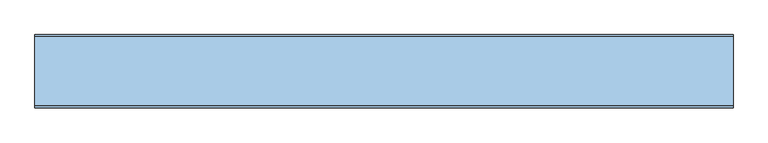
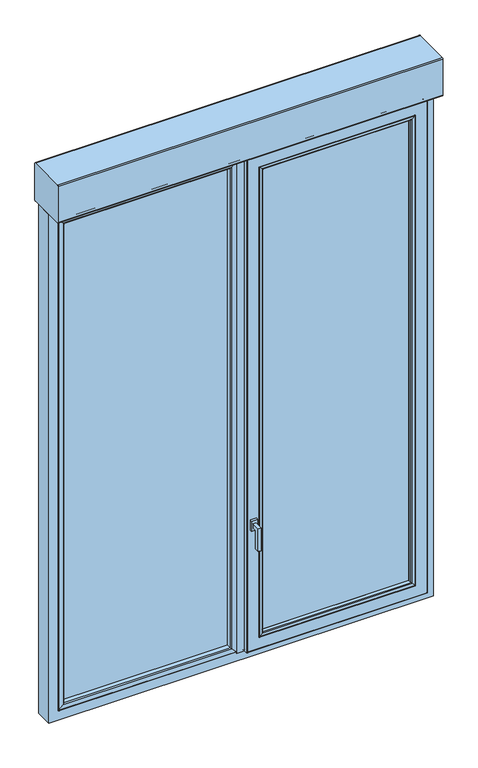
"""IFC4 building model written with IfcOpenShell, lengths in millimetres: window geometry, 2019_ES_Ventana_Replus_re80pvc301_11103_box_1-Hoja_Panel-Fijo-Lateral_con-Compacto : Salla."""

from ifc_helpers import new_model, si_unit, point, frame, frame_2d, origin, place, context, project, spatial, polyline, circle_curve, ellipse_curve, trimmed, segment, composite_curve, outline, extrude, source, transform, mapped, element, save
from ifc_brep_helpers import plane_surface, cylinder_surface, advanced_brep


def window_b88c883a(model_context):
    return source(origin(), model_context, "Body", "SolidModel", [
        extrude(outline(composite_curve([segment(polyline([(55.0, 3270.0), (-120.0, 3270.0)]), True, "CONTINUOUS"), segment(trimmed(circle_curve(frame_2d((-120.0, 3275.0)), 5.0), [point((-120.0, 3270.0))], [point((-125.0, 3275.0))], False, "CARTESIAN"), True, "CONTINUOUS"), segment(polyline([(-125.0, 3275.0), (-125.0, 3450.0)]), True, "CONTINUOUS"), segment(trimmed(circle_curve(frame_2d((-120.0, 3450.0)), 5.0), [point((-125.0, 3450.0))], [point((-120.0, 3455.0))], False, "CARTESIAN"), True, "CONTINUOUS"), segment(polyline([(-120.0, 3455.0), (55.0, 3455.0)]), True, "CONTINUOUS"), segment(trimmed(circle_curve(frame_2d((55.0, 3450.0)), 5.0), [point((55.0, 3455.0))], [point((60.0, 3450.0))], False, "CARTESIAN"), True, "CONTINUOUS"), segment(polyline([(60.0, 3450.0), (60.0, 3275.0)]), True, "CONTINUOUS"), segment(trimmed(circle_curve(frame_2d((55.0, 3275.0)), 5.0), [point((60.0, 3275.0))], [point((55.0, 3270.0))], False, "CARTESIAN"), True, "CONTINUOUS")], self_intersect=False)), frame((-880.0, 0.0, 0.0), z_axis=(1.0, 0.0, 0.0), x_axis=(0.0, 1.0, 0.0)), (0.0, 0.0, 1.0), 1760.0),
        extrude(outline(polyline([(-78.4999991, 1470.0), (-78.4999991, 1450.0), (-98.4999991, 1450.0), (-98.4999991, 1360.0), (-118.4999991, 1360.0), (-118.4999991, 1470.0), (-78.4999991, 1470.0)])), frame((38.5, 0.0, 0.0), z_axis=(1.0, 0.0, 0.0), x_axis=(0.0, 1.0, 0.0)), (0.0, 0.0, 1.0), 12.0),
        extrude(outline(polyline([(58.7312385, -78.4999991), (30.2687615, -78.4999991), (30.2687615, -68.4999991), (58.7312385, -68.4999991), (58.7312385, -78.4999991)])), frame((0.0, 0.0, 1435.217127), z_axis=(0.0, 0.0, 1.0), x_axis=(1.0, 0.0, 0.0)), (0.0, 0.0, 1.0), 49.565746),
        extrude(outline(polyline([(-37.0063666, 11.4999962), (-37.0063666, 7.4999962), (-814.1891471, 7.4999962), (-814.1891471, 11.4999962), (-37.0063666, 11.4999962)])), frame((0.0, 0.0, 875.6108529), z_axis=(0.0, 0.0, 1.0), x_axis=(1.0, 0.0, 0.0)), (0.0, 0.0, 1.0), 2328.7782941),
        extrude(outline(polyline([(-37.0063666, -6.5), (-37.0063666, -10.5), (-814.1891471, -10.5), (-814.1891471, -6.5), (-37.0063666, -6.5)])), frame((0.0, 0.0, 875.6108529), z_axis=(0.0, 0.0, 1.0), x_axis=(1.0, 0.0, 0.0)), (0.0, 0.0, 1.0), 2328.7782941),
        extrude(outline(polyline([(-37.0063666, -24.4999997), (-37.0063666, -28.4999997), (-814.1891471, -28.4999997), (-814.1891471, -24.4999997), (-37.0063666, -24.4999997)])), frame((0.0, 0.0, 875.6108529), z_axis=(0.0, 0.0, 1.0), x_axis=(1.0, 0.0, 0.0)), (0.0, 0.0, 1.0), 2328.7782941),
        advanced_brep(
        [(-22.1502489, -49.9816666, 3224.0497511), (-41.8192398, -49.2838062, 3204.3807602), (-41.8192398, -49.2838062, 875.6192398), (-22.1502489, -49.9816666, 855.9502489), (-46.4697163, -45.5846502, 3199.7302837), (-46.4697163, -45.5846502, 880.2697163), (-814.3807594, -49.2838062, 875.6192398), (-834.0497503, -49.9816666, 855.9502489), (-21.0, -48.871505, 3225.2), (-21.0, -48.871505, 854.8), (-51.0475336, -28.5000036, 3195.1524664), (-51.0475336, -28.5000036, 884.8475336), (-809.7302829, -45.5846502, 880.2697163), (-43.2922784, -28.5000036, 877.0922784), (-812.9077208, -28.5000036, 877.0922784), (-812.9077208, -28.5000036, 3202.9077216), (-43.2922784, -28.5000036, 3202.9077216), (-805.1524657, -28.5000036, 3195.1524664), (-805.1524657, -28.5000036, 884.8475336), (-35.4855, -36.306782, 3210.7145), (-35.4855, -36.306782, 869.2855), (-35.4855, -39.5069121, 3210.7145), (-35.4855, -39.5069121, 869.2855), (-820.7144993, -36.306782, 869.2855), (-21.0, -39.5069121, 854.8), (-835.1999993, -39.5069121, 854.8), (-835.1999993, -39.5069121, 3225.2), (-21.0, -39.5069121, 3225.2), (-820.7144993, -39.5069121, 3210.7145), (-820.7144993, -39.5069121, 869.2855), (-835.1999993, -48.871505, 854.8), (-814.3807594, -49.2838062, 3204.3807602), (-834.0497503, -49.9816666, 3224.0497511), (-809.7302829, -45.5846502, 3199.7302837), (-820.7144993, -36.306782, 3210.7145), (-835.1999993, -48.871505, 3225.2)],
        [
            (0, 1),
            (1, 2),
            (2, 3),
            (3, 0),
            (1, 4, ellipse_curve(frame((-41.6449168, -44.2918491, 3204.5550832), z_axis=(0.7071067811865475, 0.0, -0.7071067811865475), x_axis=(0.7071067811865474, 0.0, 0.7071067811865476)), 7.0639967, 4.995)),
            (4, 5),
            (5, 2, ellipse_curve(frame((-41.6449168, -44.2918491, 875.4449168), z_axis=(0.7071067811865475, 0.0, 0.7071067811865475), x_axis=(-0.7071067811865474, 0.0, 0.7071067811865476)), 7.0639967, 4.995)),
            (2, 6),
            (6, 7),
            (7, 3),
            (8, 0, ellipse_curve(frame((-22.1108601, -48.871505, 3224.0891399), z_axis=(0.7071067811865475, 0.0, -0.7071067811865475), x_axis=(0.7071067811865474, 0.0, 0.7071067811865476)), 1.5709935, 1.1108601)),
            (3, 9, ellipse_curve(frame((-22.1108601, -48.871505, 855.9108601), z_axis=(0.7071067811865475, 0.0, 0.7071067811865475), x_axis=(-0.7071067811865474, 0.0, 0.7071067811865476)), 1.5709935, 1.1108601)),
            (9, 8),
            (4, 10),
            (10, 11),
            (11, 5),
            (5, 12),
            (12, 6, ellipse_curve(frame((-814.5550824, -44.2918491, 875.4449168), z_axis=(0.7071067811865475, 0.0, -0.7071067811865475), x_axis=(0.7071067811865476, 0.0, 0.7071067811865474)), 7.0639967, 4.995)),
            (13, 14),
            (14, 15),
            (15, 16),
            (16, 13),
            (10, 17),
            (17, 18),
            (18, 11),
            (18, 12),
            (16, 19),
            (19, 20),
            (20, 13),
            (19, 21),
            (21, 22),
            (22, 20),
            (20, 23),
            (23, 14),
            (24, 25),
            (25, 26),
            (26, 27),
            (27, 24),
            (21, 28),
            (28, 29),
            (29, 22),
            (29, 23),
            (9, 24),
            (27, 8),
            (9, 30),
            (30, 25),
            (7, 30, ellipse_curve(frame((-834.0891391, -48.871505, 855.9108601), z_axis=(0.7071067811865475, 0.0, -0.7071067811865475), x_axis=(0.7071067811865476, 0.0, 0.7071067811865474)), 1.5709935, 1.1108601)),
            (6, 31),
            (31, 32),
            (32, 7),
            (12, 33),
            (33, 31, ellipse_curve(frame((-814.5550824, -44.2918491, 3204.5550832), z_axis=(-0.7071067811865475, 0.0, -0.7071067811865475), x_axis=(0.7071067811865474, 0.0, -0.7071067811865476)), 7.0639967, 4.995)),
            (17, 33),
            (23, 34),
            (34, 15),
            (28, 34),
            (30, 35),
            (35, 26),
            (32, 35, ellipse_curve(frame((-834.0891391, -48.871505, 3224.0891399), z_axis=(-0.7071067811865475, 0.0, -0.7071067811865475), x_axis=(0.7071067811865474, 0.0, -0.7071067811865476)), 1.5709935, 1.1108601)),
            (31, 1),
            (0, 32),
            (33, 4),
            (34, 19),
            (35, 8),
        ],
        [
            plane_surface(frame((-41.8192398, -49.2838062, 3204.3807602), z_axis=(-0.03545791932093311, -0.9993711702652975, 0.0), x_axis=(0.0, 0.0, -1.0))),
            cylinder_surface(frame((-41.6449168, -44.2918491, 3232.2), z_axis=(0.0, 0.0, 1.0), x_axis=(-1.0, 0.0, 0.0)), 4.995),
            plane_surface(frame((-41.8192398, -49.2838062, 875.6192398), z_axis=(0.0, -0.9993711702652976, 0.035457919320929884), x_axis=(-1.0, 0.0, 0.0))),
            cylinder_surface(frame((-22.1108601, -48.871505, 3232.2), z_axis=(0.0, 0.0, 1.0), x_axis=(-1.0, 0.0, 0.0)), 1.1108601),
            plane_surface(frame((-51.0475336, -28.5000036, 3195.1524664), z_axis=(-0.9659258262890619, -0.25881904510254483, 0.0), x_axis=(0.0, 0.0, -1.0))),
            cylinder_surface(frame((-14.0, -44.2918491, 875.4449168), z_axis=(1.0, 0.0, 0.0), x_axis=(0.0, 0.0, 1.0)), 4.995),
            plane_surface(frame((-812.9077208, -28.5000036, 3202.9077216), z_axis=(0.0, 1.0, 0.0), x_axis=(1.0, 0.0, 0.0))),
            plane_surface(frame((-51.0475336, -28.5000036, 884.8475336), z_axis=(0.0, -0.25881904510254794, 0.965925826289061), x_axis=(-1.0, 0.0, 0.0))),
            plane_surface(frame((-35.4855, -36.306782, 3210.7145), z_axis=(0.7071067811865617, 0.7071067811865334, 0.0), x_axis=(0.0, 0.0, -1.0))),
            plane_surface(frame((-35.4855, -39.5069121, 3210.7145), z_axis=(1.0, 0.0, 0.0), x_axis=(0.0, 0.0, -1.0))),
            plane_surface(frame((-35.4855, -36.306782, 869.2855), z_axis=(0.0, 0.7071067811865357, -0.7071067811865593), x_axis=(-1.0, 0.0, 0.0))),
            plane_surface(frame((-835.1999993, -39.5069121, 3225.2), z_axis=(0.0, 1.0, 0.0), x_axis=(1.0, 0.0, 0.0))),
            plane_surface(frame((-35.4855, -39.5069121, 869.2855), z_axis=(0.0, 0.0, -1.0), x_axis=(-1.0, 0.0, 0.0))),
            plane_surface(frame((-21.0, -46.2002121, 3225.2), z_axis=(1.0, 0.0, 0.0), x_axis=(0.0, 0.0, -1.0))),
            plane_surface(frame((-21.0, -46.2002121, 854.8), z_axis=(0.0, 0.0, -1.0), x_axis=(-1.0, 0.0, 0.0))),
            cylinder_surface(frame((-14.0, -48.871505, 855.9108601), z_axis=(1.0, 0.0, 0.0), x_axis=(0.0, 0.0, 1.0)), 1.1108601),
            plane_surface(frame((-814.3807594, -49.2838062, 875.6192398), z_axis=(0.03545791932092666, -0.9993711702652978, 0.0), x_axis=(0.0, 0.0, 1.0))),
            cylinder_surface(frame((-814.5550824, -44.2918491, 847.8), z_axis=(0.0, 0.0, -1.0), x_axis=(1.0, 0.0, 0.0)), 4.995),
            plane_surface(frame((-805.1524657, -28.5000036, 884.8475336), z_axis=(0.9659258262890602, -0.2588190451025511, 0.0), x_axis=(0.0, 0.0, 1.0))),
            plane_surface(frame((-820.7144993, -36.306782, 869.2855), z_axis=(-0.707106781186557, 0.707106781186538, 0.0), x_axis=(0.0, 0.0, 1.0))),
            plane_surface(frame((-820.7144993, -39.5069121, 869.2855), z_axis=(-1.0, 0.0, 0.0), x_axis=(0.0, 0.0, 1.0))),
            plane_surface(frame((-835.1999993, -46.2002121, 854.8), z_axis=(-1.0, 0.0, 0.0), x_axis=(0.0, 0.0, 1.0))),
            cylinder_surface(frame((-834.0891391, -48.871505, 847.8), z_axis=(0.0, 0.0, -1.0), x_axis=(1.0, 0.0, 0.0)), 1.1108601),
            plane_surface(frame((-814.3807594, -49.2838062, 3204.3807602), z_axis=(0.0, -0.9993711702652976, -0.035457919320929884), x_axis=(1.0, 0.0, 0.0))),
            cylinder_surface(frame((-842.1999993, -44.2918491, 3204.5550832), z_axis=(-1.0, 0.0, 0.0), x_axis=(0.0, 0.0, -1.0)), 4.995),
            plane_surface(frame((-805.1524657, -28.5000036, 3195.1524664), z_axis=(0.0, -0.258819045102548, -0.9659258262890611), x_axis=(1.0, 0.0, 0.0))),
            plane_surface(frame((-820.7144993, -36.306782, 3210.7145), z_axis=(0.0, 0.7071067811865357, 0.7071067811865593), x_axis=(1.0, 0.0, 0.0))),
            plane_surface(frame((-820.7144993, -39.5069121, 3210.7145), z_axis=(0.0, 0.0, 1.0), x_axis=(1.0, 0.0, 0.0))),
            plane_surface(frame((-835.1999993, -46.2002121, 3225.2), z_axis=(0.0, 0.0, 1.0), x_axis=(1.0, 0.0, 0.0))),
            cylinder_surface(frame((-842.1999993, -48.871505, 3224.0891399), z_axis=(-1.0, 0.0, 0.0), x_axis=(0.0, 0.0, -1.0)), 1.1108601),
        ],
        [
            (0, [[1, 2, 3, 4]]),
            (1, [[5, 6, 7, -2]]),
            (2, [[-3, 8, 9, 10]]),
            (3, [[11, -4, 12, 13]]),
            (4, [[14, 15, 16, -6]]),
            (5, [[-7, 17, 18, -8]]),
            (6, [[19, 20, 21, 22], [23, 24, 25, -15]]),
            (7, [[-16, -25, 26, -17]]),
            (8, [[27, 28, 29, -22]]),
            (9, [[30, 31, 32, -28]]),
            (10, [[-29, 33, 34, -19]]),
            (11, [[35, 36, 37, 38], [39, 40, 41, -31]]),
            (12, [[-32, -41, 42, -33]]),
            (13, [[-13, 43, -38, 44]]),
            (14, [[-43, 45, 46, -35]]),
            (15, [[-12, -10, 47, -45]]),
            (16, [[-9, 48, 49, 50]]),
            (17, [[-18, 51, 52, -48]]),
            (18, [[-26, -24, 53, -51]]),
            (19, [[-34, 54, 55, -20]]),
            (20, [[-42, -40, 56, -54]]),
            (21, [[-46, 57, 58, -36]]),
            (22, [[-47, -50, 59, -57]]),
            (23, [[-49, 60, -1, 61]]),
            (24, [[-52, 62, -5, -60]]),
            (25, [[-53, -23, -14, -62]]),
            (26, [[-55, 63, -27, -21]]),
            (27, [[-56, -39, -30, -63]]),
            (28, [[-58, 64, -44, -37]]),
            (29, [[-59, -61, -11, -64]]),
        ],
    ),
        extrude(outline(polyline([(3167.0, 777.1999993), (3167.0, 81.0), (912.8, 81.0), (912.8, 777.1999993), (3167.0, 777.1999993)]), holes=[polyline([(920.8, 769.1999993), (920.8, 89.0), (3159.0, 89.0), (3159.0, 769.1999993), (920.8, 769.1999993)])]), frame((0.0, -27.0000002, 0.0), z_axis=(0.0, 1.0, 0.0), x_axis=(0.0, 0.0, 1.0)), (0.0, 0.0, 1.0), 16.0000002),
        extrude(outline(polyline([(3167.0, 777.1999993), (3167.0, 81.0), (912.8, 81.0), (912.8, 777.1999993), (3167.0, 777.1999993)]), holes=[polyline([(920.8, 769.1999993), (920.8, 89.0), (3159.0, 89.0), (3159.0, 769.1999993), (920.8, 769.1999993)])]), frame((0.0, -47.0000002, 0.0), z_axis=(0.0, 1.0, 0.0), x_axis=(0.0, 0.0, 1.0)), (0.0, 0.0, 1.0), 16.0000002),
        extrude(outline(polyline([(3198.3891471, -43.0063666), (3198.3891471, -808.1891471), (881.8608529, -808.1891471), (881.8608529, -43.0063666), (3198.3891471, -43.0063666)]), holes=[polyline([(889.8608529, -51.0063666), (889.8608529, -800.1891471), (3190.3891471, -800.1891471), (3190.3891471, -51.0063666), (889.8608529, -51.0063666)])]), frame((0.0, -24.5, 0.0), z_axis=(0.0, 1.0, 0.0), x_axis=(0.0, 0.0, 1.0)), (0.0, 0.0, 1.0), 14.0),
        extrude(outline(polyline([(3198.3891471, -43.0063666), (3198.3891471, -808.1891471), (881.8608529, -808.1891471), (881.8608529, -43.0063666), (3198.3891471, -43.0063666)]), holes=[polyline([(889.8608529, -51.0063666), (889.8608529, -800.1891471), (3190.3891471, -800.1891471), (3190.3891471, -51.0063666), (889.8608529, -51.0063666)])]), frame((0.0, -6.5, 0.0), z_axis=(0.0, 1.0, 0.0), x_axis=(0.0, 0.0, 1.0)), (0.0, 0.0, 1.0), 14.0),
        advanced_brep(
        [(48.1911809, 11.5, 3200.2), (48.1911809, 11.5, 879.8), (48.1911809, -11.9999991, 879.8), (48.1911809, -11.9999991, 3200.2), (810.1999993, 11.5, 3200.2), (810.1999993, 11.5, 879.8), (88.2020856, 11.5, 919.8109047), (770.1890945, 11.5, 919.8109047), (770.1890945, 11.5, 3160.1890953), (88.2020856, 11.5, 3160.1890953), (810.1999993, -11.9999991, 879.8), (35.1911809, -11.9999991, 3213.2), (823.1999993, -11.9999991, 3213.2), (823.1999993, -11.9999991, 866.8), (35.1911809, -11.9999991, 866.8), (810.1999993, -11.9999991, 3200.2), (35.1911809, -50.0, 866.8), (35.1911809, -50.0, 3213.2), (823.1999993, -50.0, 866.8), (15.1911809, -50.0, 3233.2), (843.1999993, -50.0, 3233.2), (843.1999993, -50.0, 846.8), (15.1911809, -50.0, 846.8), (823.1999993, -50.0, 3213.2), (15.1911809, -65.4999991, 3233.2), (15.1911809, -65.4999991, 846.8), (843.1999993, -65.4999991, 846.8), (18.1911809, -68.4999991, 3230.2), (18.1911809, -68.4999991, 849.8), (840.1999993, -68.4999991, 849.8), (840.1999993, -68.4999991, 3230.2), (70.9541209, -68.4999991, 3177.43706), (787.4370593, -68.4999991, 3177.43706), (787.4370593, -68.4999991, 902.56294), (70.9541209, -68.4999991, 902.56294), (72.1911809, -67.2629391, 3176.2), (72.1911809, -67.2629391, 903.8), (786.1999993, -67.2629391, 903.8), (72.7423375, -67.7951848, 3175.6488434), (72.7423375, -67.7951848, 904.3511566), (785.6488427, -67.7951848, 904.3511566), (85.7676831, -67.3403297, 3162.6234978), (85.7676831, -67.3403297, 917.3765022), (772.6234971, -67.3403297, 917.3765022), (89.4917884, -64.3780426, 3158.8993925), (89.4917884, -64.3780426, 921.1006075), (768.8993918, -64.3780426, 921.1006075), (92.8970803, -51.6693201, 3155.4941006), (92.8970803, -51.6693201, 924.5058994), (765.4940999, -51.6693201, 924.5058994), (92.3834932, -51.0000003, 3156.0076877), (92.3834932, -51.0000003, 923.9923123), (766.007687, -51.0000003, 923.9923123), (81.1911809, -51.0000003, 3167.2), (777.1999993, -51.0000003, 3167.2), (777.1999993, -51.0000003, 912.8), (81.1911809, -51.0000003, 912.8), (766.007687, -51.0000003, 3156.0076877), (81.1911809, -56.4999995, 3167.2), (81.1911809, -56.4999995, 912.8), (777.1999993, -56.4999995, 912.8), (69.1911809, -56.4999995, 3179.2), (789.1999993, -56.4999995, 3179.2), (789.1999993, -56.4999995, 900.8), (69.1911809, -56.4999995, 900.8), (777.1999993, -56.4999995, 3167.2), (69.1911809, -25.6153717, 3179.2), (69.1911809, -25.6153717, 900.8), (789.1999993, -25.6153717, 900.8), (66.574961, -6.9999997, 3181.8162199), (66.574961, -6.9999997, 898.1837801), (791.8162192, -6.9999997, 898.1837801), (791.8162192, -6.9999997, 3181.8162199), (87.1911809, -6.9999997, 3161.2), (771.1999993, -6.9999997, 3161.2), (771.1999993, -6.9999997, 918.8), (87.1911809, -6.9999997, 918.8), (87.1911809, -3.0000033, 3161.2), (87.1911809, -3.0000033, 918.8), (771.1999993, -3.0000033, 918.8), (771.1999993, -3.0000033, 3161.2), (93.7172496, -3.0000033, 3154.6739313), (764.6739305, -3.0000033, 3154.6739313), (764.6739305, -3.0000033, 925.3260687), (93.7172496, -3.0000033, 925.3260687), (94.2153834, -2.3508228, 3154.1757976), (94.2153834, -2.3508228, 925.8242024), (764.1757968, -2.3508228, 925.8242024), (91.0998631, 9.2764571, 3157.2913178), (91.0998631, 9.2764571, 922.7086822), (767.2913171, 9.2764571, 922.7086822), (843.1999993, -65.4999991, 3233.2), (786.1999993, -67.2629391, 3176.2), (785.6488427, -67.7951848, 3175.6488434), (772.6234971, -67.3403297, 3162.6234978), (768.8993918, -64.3780426, 3158.8993925), (765.4940999, -51.6693201, 3155.4941006), (789.1999993, -25.6153717, 3179.2), (764.1757968, -2.3508228, 3154.1757976), (767.2913171, 9.2764571, 3157.2913178)],
        [
            (0, 1),
            (1, 2),
            (2, 3),
            (3, 0),
            (0, 4),
            (4, 5),
            (5, 1),
            (6, 7),
            (7, 8),
            (8, 9),
            (9, 6),
            (5, 10),
            (10, 2),
            (11, 12),
            (12, 13),
            (13, 14),
            (14, 11),
            (10, 15),
            (15, 3),
            (14, 16),
            (16, 17),
            (17, 11),
            (13, 18),
            (18, 16),
            (19, 20),
            (20, 21),
            (21, 22),
            (22, 19),
            (18, 23),
            (23, 17),
            (24, 19),
            (22, 25),
            (25, 24),
            (21, 26),
            (26, 25),
            (27, 24, ellipse_curve(frame((18.1911809, -65.4999991, 3230.2), z_axis=(-0.7071067811865475, 0.0, -0.7071067811865475), x_axis=(-0.7071067811865474, 0.0, 0.7071067811865476)), 4.2426407, 3.0)),
            (25, 28, ellipse_curve(frame((18.1911809, -65.4999991, 849.8), z_axis=(-0.7071067811865475, 0.0, 0.7071067811865475), x_axis=(0.7071067811865474, 0.0, 0.7071067811865476)), 4.2426407, 3.0)),
            (28, 27),
            (26, 29, ellipse_curve(frame((840.1999993, -65.4999991, 849.8), z_axis=(-0.7071067811865475, 0.0, -0.7071067811865475), x_axis=(-0.7071067811865476, 0.0, 0.7071067811865474)), 4.2426407, 3.0)),
            (29, 28),
            (29, 30),
            (30, 27),
            (31, 32),
            (32, 33),
            (33, 34),
            (34, 31),
            (35, 31, ellipse_curve(frame((70.9541209, -67.2629391, 3177.43706), z_axis=(-0.7071067811865475, 0.0, -0.7071067811865475), x_axis=(-0.7071067811865474, 0.0, 0.7071067811865476)), 1.7494671, 1.23706)),
            (34, 36, ellipse_curve(frame((70.9541209, -67.2629391, 902.56294), z_axis=(-0.7071067811865475, 0.0, 0.7071067811865475), x_axis=(0.7071067811865474, 0.0, 0.7071067811865476)), 1.7494671, 1.23706)),
            (36, 35),
            (33, 37, ellipse_curve(frame((787.4370593, -67.2629391, 902.56294), z_axis=(-0.7071067811865475, 0.0, -0.7071067811865475), x_axis=(-0.7071067811865476, 0.0, 0.7071067811865474)), 1.7494671, 1.23706)),
            (37, 36),
            (38, 35, ellipse_curve(frame((72.7237511, -67.2629391, 3175.6674299), z_axis=(-0.7071067811865475, 0.0, -0.7071067811865475), x_axis=(-0.7071067811865474, 0.0, 0.7071067811865476)), 0.7531679, 0.5325701)),
            (36, 39, ellipse_curve(frame((72.7237511, -67.2629391, 904.3325701), z_axis=(-0.7071067811865475, 0.0, 0.7071067811865475), x_axis=(0.7071067811865474, 0.0, 0.7071067811865476)), 0.7531679, 0.5325701)),
            (39, 38),
            (37, 40, ellipse_curve(frame((785.6674291, -67.2629391, 904.3325701), z_axis=(-0.7071067811865475, 0.0, -0.7071067811865475), x_axis=(-0.7071067811865476, 0.0, 0.7071067811865474)), 0.7531679, 0.5325701)),
            (40, 39),
            (41, 38),
            (39, 42),
            (42, 41),
            (40, 43),
            (43, 42),
            (44, 41, ellipse_curve(frame((85.6280851, -63.3427664, 3162.7630958), z_axis=(-0.7071067811865475, 0.0, -0.7071067811865475), x_axis=(-0.7071067811865474, 0.0, 0.7071067811865476)), 5.6568542, 4.0)),
            (42, 45, ellipse_curve(frame((85.6280851, -63.3427664, 917.2369042), z_axis=(-0.7071067811865475, 0.0, 0.7071067811865475), x_axis=(0.7071067811865474, 0.0, 0.7071067811865476)), 5.6568542, 4.0)),
            (45, 44),
            (43, 46, ellipse_curve(frame((772.7630951, -63.3427664, 917.2369042), z_axis=(-0.7071067811865475, 0.0, -0.7071067811865475), x_axis=(-0.7071067811865476, 0.0, 0.7071067811865474)), 5.6568542, 4.0)),
            (46, 45),
            (47, 44),
            (45, 48),
            (48, 47),
            (46, 49),
            (49, 48),
            (50, 47, ellipse_curve(frame((92.3834932, -51.5317048, 3156.0076877), z_axis=(-0.7071067811865475, 0.0, -0.7071067811865475), x_axis=(-0.7071067811865474, 0.0, 0.7071067811865476)), 0.7519437, 0.5317045)),
            (48, 51, ellipse_curve(frame((92.3834932, -51.5317048, 923.9923123), z_axis=(-0.7071067811865475, 0.0, 0.7071067811865475), x_axis=(0.7071067811865474, 0.0, 0.7071067811865476)), 0.7519437, 0.5317045)),
            (51, 50),
            (49, 52, ellipse_curve(frame((766.007687, -51.5317048, 923.9923123), z_axis=(-0.7071067811865475, 0.0, -0.7071067811865475), x_axis=(-0.7071067811865476, 0.0, 0.7071067811865474)), 0.7519437, 0.5317045)),
            (52, 51),
            (53, 54),
            (54, 55),
            (55, 56),
            (56, 53),
            (52, 57),
            (57, 50),
            (58, 53),
            (56, 59),
            (59, 58),
            (55, 60),
            (60, 59),
            (61, 62),
            (62, 63),
            (63, 64),
            (64, 61),
            (60, 65),
            (65, 58),
            (66, 61),
            (64, 67),
            (67, 66),
            (63, 68),
            (68, 67),
            (69, 66),
            (67, 70),
            (70, 69),
            (68, 71),
            (71, 70),
            (71, 72),
            (72, 69),
            (73, 74),
            (74, 75),
            (75, 76),
            (76, 73),
            (77, 73),
            (76, 78),
            (78, 77),
            (75, 79),
            (79, 78),
            (79, 80),
            (80, 77),
            (81, 82),
            (82, 83),
            (83, 84),
            (84, 81),
            (85, 81, ellipse_curve(frame((93.7172496, -2.4842973, 3154.6739313), z_axis=(-0.7071067811865475, 0.0, -0.7071067811865475), x_axis=(-0.7071067811865474, 0.0, 0.7071067811865476)), 0.7293184, 0.515706)),
            (84, 86, ellipse_curve(frame((93.7172496, -2.4842973, 925.3260687), z_axis=(-0.7071067811865475, 0.0, 0.7071067811865475), x_axis=(0.7071067811865474, 0.0, 0.7071067811865476)), 0.7293184, 0.515706)),
            (86, 85),
            (83, 87, ellipse_curve(frame((764.6739305, -2.4842973, 925.3260687), z_axis=(-0.7071067811865475, 0.0, -0.7071067811865475), x_axis=(-0.7071067811865476, 0.0, 0.7071067811865474)), 0.7293184, 0.515706)),
            (87, 86),
            (88, 85),
            (86, 89),
            (89, 88),
            (87, 90),
            (90, 89),
            (9, 88, ellipse_curve(frame((88.2020856, 8.5, 3160.1890953), z_axis=(-0.7071067811865475, 0.0, -0.7071067811865475), x_axis=(-0.7071067811865474, 0.0, 0.7071067811865476)), 4.2426407, 3.0)),
            (89, 6, ellipse_curve(frame((88.2020856, 8.5, 919.8109047), z_axis=(-0.7071067811865475, 0.0, 0.7071067811865475), x_axis=(0.7071067811865474, 0.0, 0.7071067811865476)), 4.2426407, 3.0)),
            (90, 7, ellipse_curve(frame((770.1890945, 8.5, 919.8109047), z_axis=(-0.7071067811865475, 0.0, -0.7071067811865475), x_axis=(-0.7071067811865476, 0.0, 0.7071067811865474)), 4.2426407, 3.0)),
            (4, 15),
            (12, 23),
            (20, 91),
            (91, 26),
            (91, 30, ellipse_curve(frame((840.1999993, -65.4999991, 3230.2), z_axis=(0.7071067811865475, 0.0, -0.7071067811865475), x_axis=(-0.7071067811865474, 0.0, -0.7071067811865476)), 4.2426407, 3.0)),
            (32, 92, ellipse_curve(frame((787.4370593, -67.2629391, 3177.43706), z_axis=(0.7071067811865475, 0.0, -0.7071067811865475), x_axis=(-0.7071067811865474, 0.0, -0.7071067811865476)), 1.7494671, 1.23706)),
            (92, 37),
            (92, 93, ellipse_curve(frame((785.6674291, -67.2629391, 3175.6674299), z_axis=(0.7071067811865475, 0.0, -0.7071067811865475), x_axis=(-0.7071067811865474, 0.0, -0.7071067811865476)), 0.7531679, 0.5325701)),
            (93, 40),
            (93, 94),
            (94, 43),
            (94, 95, ellipse_curve(frame((772.7630951, -63.3427664, 3162.7630958), z_axis=(0.7071067811865475, 0.0, -0.7071067811865475), x_axis=(-0.7071067811865474, 0.0, -0.7071067811865476)), 5.6568542, 4.0)),
            (95, 46),
            (95, 96),
            (96, 49),
            (96, 57, ellipse_curve(frame((766.007687, -51.5317048, 3156.0076877), z_axis=(0.7071067811865475, 0.0, -0.7071067811865475), x_axis=(-0.7071067811865474, 0.0, -0.7071067811865476)), 0.7519437, 0.5317045)),
            (54, 65),
            (62, 97),
            (97, 68),
            (97, 72),
            (74, 80),
            (82, 98, ellipse_curve(frame((764.6739305, -2.4842973, 3154.6739313), z_axis=(0.7071067811865475, 0.0, -0.7071067811865475), x_axis=(-0.7071067811865474, 0.0, -0.7071067811865476)), 0.7293184, 0.515706)),
            (98, 87),
            (98, 99),
            (99, 90),
            (99, 8, ellipse_curve(frame((770.1890945, 8.5, 3160.1890953), z_axis=(0.7071067811865475, 0.0, -0.7071067811865475), x_axis=(-0.7071067811865474, 0.0, -0.7071067811865476)), 4.2426407, 3.0)),
            (24, 91),
            (35, 92),
            (38, 93),
            (41, 94),
            (44, 95),
            (47, 96),
            (66, 97),
            (85, 98),
            (88, 99),
        ],
        [
            plane_surface(frame((48.1911809, -1.4999991, 3200.2), z_axis=(-1.0, 0.0, 0.0), x_axis=(0.0, 0.0, -1.0))),
            plane_surface(frame((770.1890945, 11.5, 3160.1890953), z_axis=(0.0, 1.0, 0.0), x_axis=(-1.0, 0.0, 0.0))),
            plane_surface(frame((48.1911809, -1.4999991, 879.8), z_axis=(0.0, 0.0, -1.0), x_axis=(1.0, 0.0, 0.0))),
            plane_surface(frame((815.7000002, -11.9999991, 3205.7000009), z_axis=(0.0, 1.0, 0.0), x_axis=(-1.0, 0.0, 0.0))),
            plane_surface(frame((35.1911809, -45.0999991, 3213.2), z_axis=(-1.0, 0.0, 0.0), x_axis=(0.0, 0.0, -1.0))),
            plane_surface(frame((35.1911809, -45.0999991, 866.8), z_axis=(0.0, 0.0, -1.0), x_axis=(1.0, 0.0, 0.0))),
            plane_surface(frame((839.2000019, -50.0, 3229.2000027), z_axis=(0.0, 1.0, 0.0), x_axis=(-1.0, 0.0, 0.0))),
            plane_surface(frame((15.1911809, -50.0, 3233.2), z_axis=(-1.0, 0.0, 0.0), x_axis=(0.0, 0.0, -1.0))),
            plane_surface(frame((15.1911809, -50.0, 846.8), z_axis=(0.0, 0.0, -1.0), x_axis=(1.0, 0.0, 0.0))),
            cylinder_surface(frame((18.1911809, -65.4999991, 3233.2), z_axis=(0.0, 0.0, 1.0), x_axis=(0.0, 1.0, 0.0)), 3.0),
            cylinder_surface(frame((15.1911809, -65.4999991, 849.8), z_axis=(-1.0, 0.0, 0.0), x_axis=(0.0, 1.0, 0.0)), 3.0),
            plane_surface(frame((840.1999993, -68.4999991, 3230.2), z_axis=(0.0, -1.0, 0.0), x_axis=(-1.0, 0.0, 0.0))),
            cylinder_surface(frame((70.9541209, -67.2629391, 3233.2), z_axis=(0.0, 0.0, 1.0), x_axis=(0.0, 1.0, 0.0)), 1.23706),
            cylinder_surface(frame((15.1911809, -67.2629391, 902.56294), z_axis=(-1.0, 0.0, 0.0), x_axis=(0.0, 1.0, 0.0)), 1.23706),
            cylinder_surface(frame((72.7237511, -67.2629391, 3233.2), z_axis=(0.0, 0.0, 1.0), x_axis=(0.0, 1.0, 0.0)), 0.5325701),
            cylinder_surface(frame((15.1911809, -67.2629391, 904.3325701), z_axis=(-1.0, 0.0, 0.0), x_axis=(0.0, 1.0, 0.0)), 0.5325701),
            plane_surface(frame((72.7423375, -67.7951848, 3175.6488434), z_axis=(0.03489949670249966, -0.9993908270190959, 0.0), x_axis=(0.0, 0.0, -1.0))),
            plane_surface(frame((72.7423375, -67.7951848, 904.3511566), z_axis=(0.0, -0.9993908270190958, 0.034899496702502884), x_axis=(1.0, 0.0, 0.0))),
            cylinder_surface(frame((85.6280851, -63.3427664, 3233.2), z_axis=(0.0, 0.0, 1.0), x_axis=(0.0, 1.0, 0.0)), 4.0),
            cylinder_surface(frame((15.1911809, -63.3427664, 917.2369042), z_axis=(-1.0, 0.0, 0.0), x_axis=(0.0, 1.0, 0.0)), 4.0),
            plane_surface(frame((89.4917884, -64.3780426, 3158.8993925), z_axis=(0.9659258262890643, -0.2588190451025359, 0.0), x_axis=(0.0, 0.0, -1.0))),
            plane_surface(frame((89.4917884, -64.3780426, 921.1006075), z_axis=(0.0, -0.2588190451025328, 0.9659258262890652), x_axis=(1.0, 0.0, 0.0))),
            cylinder_surface(frame((92.3834932, -51.5317048, 3233.2), z_axis=(0.0, 0.0, 1.0), x_axis=(0.0, 1.0, 0.0)), 0.5317045),
            cylinder_surface(frame((15.1911809, -51.5317048, 923.9923123), z_axis=(-1.0, 0.0, 0.0), x_axis=(0.0, 1.0, 0.0)), 0.5317045),
            plane_surface(frame((766.007687, -51.0000003, 3156.0076877), z_axis=(0.0, 1.0, 0.0), x_axis=(-1.0, 0.0, 0.0))),
            plane_surface(frame((81.1911809, -51.0000003, 3167.2), z_axis=(-1.0, 0.0, 0.0), x_axis=(0.0, 0.0, -1.0))),
            plane_surface(frame((81.1911809, -51.0000003, 912.8), z_axis=(0.0, 0.0, -1.0), x_axis=(1.0, 0.0, 0.0))),
            plane_surface(frame((777.1999993, -56.4999995, 3167.2), z_axis=(0.0, 1.0, 0.0), x_axis=(-1.0, 0.0, 0.0))),
            plane_surface(frame((69.1911809, -56.4999995, 3179.2), z_axis=(1.0, 0.0, 0.0), x_axis=(0.0, 0.0, -1.0))),
            plane_surface(frame((69.1911809, -56.4999995, 900.8), z_axis=(0.0, 0.0, 1.0), x_axis=(1.0, 0.0, 0.0))),
            plane_surface(frame((69.1911809, -25.6153717, 3179.2), z_axis=(0.9902680687415736, 0.13917310096004257, 0.0), x_axis=(0.0, 0.0, -1.0))),
            plane_surface(frame((69.1911809, -25.6153717, 900.8), z_axis=(0.0, 0.13917310096004576, 0.9902680687415731), x_axis=(1.0, 0.0, 0.0))),
            plane_surface(frame((791.8162192, -6.9999997, 3181.8162199), z_axis=(0.0, -1.0, 0.0), x_axis=(-1.0, 0.0, 0.0))),
            plane_surface(frame((87.1911809, -6.9999997, 3161.2), z_axis=(1.0, 0.0, 0.0), x_axis=(0.0, 0.0, -1.0))),
            plane_surface(frame((87.1911809, -6.9999997, 918.8), z_axis=(0.0, 0.0, 1.0), x_axis=(1.0, 0.0, 0.0))),
            plane_surface(frame((771.1999993, -3.0000033, 3161.2), z_axis=(0.0, -1.0, 0.0), x_axis=(-1.0, 0.0, 0.0))),
            cylinder_surface(frame((93.7172496, -2.4842973, 3233.2), z_axis=(0.0, 0.0, 1.0), x_axis=(0.0, 1.0, 0.0)), 0.515706),
            cylinder_surface(frame((15.1911809, -2.4842973, 925.3260687), z_axis=(-1.0, 0.0, 0.0), x_axis=(0.0, 1.0, 0.0)), 0.515706),
            plane_surface(frame((94.2153834, -2.3508228, 3154.1757976), z_axis=(0.9659258263570589, 0.2588190448487762, 0.0), x_axis=(0.0, 0.0, -1.0))),
            plane_surface(frame((94.2153834, -2.3508228, 925.8242024), z_axis=(0.0, 0.2588190448487794, 0.9659258263570581), x_axis=(1.0, 0.0, 0.0))),
            cylinder_surface(frame((88.2020856, 8.5, 3233.2), z_axis=(0.0, 0.0, 1.0), x_axis=(0.0, 1.0, 0.0)), 3.0),
            cylinder_surface(frame((15.1911809, 8.5, 919.8109047), z_axis=(-1.0, 0.0, 0.0), x_axis=(0.0, 1.0, 0.0)), 3.0),
            plane_surface(frame((810.1999993, -1.4999991, 879.8), z_axis=(1.0, 0.0, 0.0), x_axis=(0.0, 0.0, 1.0))),
            plane_surface(frame((823.1999993, -45.0999991, 866.8), z_axis=(1.0, 0.0, 0.0), x_axis=(0.0, 0.0, 1.0))),
            plane_surface(frame((843.1999993, -50.0, 846.8), z_axis=(1.0, 0.0, 0.0), x_axis=(0.0, 0.0, 1.0))),
            cylinder_surface(frame((840.1999993, -65.4999991, 846.8), z_axis=(0.0, 0.0, -1.0), x_axis=(0.0, 1.0, 0.0)), 3.0),
            cylinder_surface(frame((787.4370593, -67.2629391, 846.8), z_axis=(0.0, 0.0, -1.0), x_axis=(0.0, 1.0, 0.0)), 1.23706),
            cylinder_surface(frame((785.6674291, -67.2629391, 846.8), z_axis=(0.0, 0.0, -1.0), x_axis=(0.0, 1.0, 0.0)), 0.5325701),
            plane_surface(frame((785.6488427, -67.7951848, 904.3511566), z_axis=(-0.03489949670250611, -0.9993908270190957, 0.0), x_axis=(0.0, 0.0, 1.0))),
            cylinder_surface(frame((772.7630951, -63.3427664, 846.8), z_axis=(0.0, 0.0, -1.0), x_axis=(0.0, 1.0, 0.0)), 4.0),
            plane_surface(frame((768.8993918, -64.3780426, 921.1006075), z_axis=(-0.965925826289066, -0.2588190451025297, 0.0), x_axis=(0.0, 0.0, 1.0))),
            cylinder_surface(frame((766.007687, -51.5317048, 846.8), z_axis=(0.0, 0.0, -1.0), x_axis=(0.0, 1.0, 0.0)), 0.5317045),
            plane_surface(frame((777.1999993, -51.0000003, 912.8), z_axis=(1.0, 0.0, 0.0), x_axis=(0.0, 0.0, 1.0))),
            plane_surface(frame((789.1999993, -56.4999995, 900.8), z_axis=(-1.0, 0.0, 0.0), x_axis=(0.0, 0.0, 1.0))),
            plane_surface(frame((789.1999993, -25.6153717, 900.8), z_axis=(-0.9902680687415727, 0.13917310096004895, 0.0), x_axis=(0.0, 0.0, 1.0))),
            plane_surface(frame((771.1999993, -6.9999997, 918.8), z_axis=(-1.0, 0.0, 0.0), x_axis=(0.0, 0.0, 1.0))),
            cylinder_surface(frame((764.6739305, -2.4842973, 846.8), z_axis=(0.0, 0.0, -1.0), x_axis=(0.0, 1.0, 0.0)), 0.515706),
            plane_surface(frame((764.1757968, -2.3508228, 925.8242024), z_axis=(-0.9659258263570573, 0.2588190448487825, 0.0), x_axis=(0.0, 0.0, 1.0))),
            cylinder_surface(frame((770.1890945, 8.5, 846.8), z_axis=(0.0, 0.0, -1.0), x_axis=(0.0, 1.0, 0.0)), 3.0),
            plane_surface(frame((810.1999993, -1.4999991, 3200.2), z_axis=(0.0, 0.0, 1.0), x_axis=(-1.0, 0.0, 0.0))),
            plane_surface(frame((823.1999993, -45.0999991, 3213.2), z_axis=(0.0, 0.0, 1.0), x_axis=(-1.0, 0.0, 0.0))),
            plane_surface(frame((843.1999993, -50.0, 3233.2), z_axis=(0.0, 0.0, 1.0), x_axis=(-1.0, 0.0, 0.0))),
            cylinder_surface(frame((843.1999993, -65.4999991, 3230.2), z_axis=(1.0, 0.0, 0.0), x_axis=(0.0, 1.0, 0.0)), 3.0),
            cylinder_surface(frame((843.1999993, -67.2629391, 3177.43706), z_axis=(1.0, 0.0, 0.0), x_axis=(0.0, 1.0, 0.0)), 1.23706),
            cylinder_surface(frame((843.1999993, -67.2629391, 3175.6674299), z_axis=(1.0, 0.0, 0.0), x_axis=(0.0, 1.0, 0.0)), 0.5325701),
            plane_surface(frame((785.6488427, -67.7951848, 3175.6488434), z_axis=(0.0, -0.9993908270190958, -0.034899496702502884), x_axis=(-1.0, 0.0, 0.0))),
            cylinder_surface(frame((843.1999993, -63.3427664, 3162.7630958), z_axis=(1.0, 0.0, 0.0), x_axis=(0.0, 1.0, 0.0)), 4.0),
            plane_surface(frame((768.8993918, -64.3780426, 3158.8993925), z_axis=(0.0, -0.2588190451025328, -0.9659258262890651), x_axis=(-1.0, 0.0, 0.0))),
            cylinder_surface(frame((843.1999993, -51.5317048, 3156.0076877), z_axis=(1.0, 0.0, 0.0), x_axis=(0.0, 1.0, 0.0)), 0.5317045),
            plane_surface(frame((777.1999993, -51.0000003, 3167.2), z_axis=(0.0, 0.0, 1.0), x_axis=(-1.0, 0.0, 0.0))),
            plane_surface(frame((789.1999993, -56.4999995, 3179.2), z_axis=(0.0, 0.0, -1.0), x_axis=(-1.0, 0.0, 0.0))),
            plane_surface(frame((789.1999993, -25.6153717, 3179.2), z_axis=(0.0, 0.13917310096004576, -0.9902680687415731), x_axis=(-1.0, 0.0, 0.0))),
            plane_surface(frame((771.1999993, -6.9999997, 3161.2), z_axis=(0.0, 0.0, -1.0), x_axis=(-1.0, 0.0, 0.0))),
            cylinder_surface(frame((843.1999993, -2.4842973, 3154.6739313), z_axis=(1.0, 0.0, 0.0), x_axis=(0.0, 1.0, 0.0)), 0.515706),
            plane_surface(frame((764.1757968, -2.3508228, 3154.1757976), z_axis=(0.0, 0.2588190448487794, -0.9659258263570581), x_axis=(-1.0, 0.0, 0.0))),
            cylinder_surface(frame((843.1999993, 8.5, 3160.1890953), z_axis=(1.0, 0.0, 0.0), x_axis=(0.0, 1.0, 0.0)), 3.0),
        ],
        [
            (0, [[1, 2, 3, 4]]),
            (1, [[5, 6, 7, -1], [8, 9, 10, 11]]),
            (2, [[-2, -7, 12, 13]]),
            (3, [[14, 15, 16, 17], [-13, 18, 19, -3]]),
            (4, [[-17, 20, 21, 22]]),
            (5, [[-20, -16, 23, 24]]),
            (6, [[25, 26, 27, 28], [-24, 29, 30, -21]]),
            (7, [[31, -28, 32, 33]]),
            (8, [[-32, -27, 34, 35]]),
            (9, [[36, -33, 37, 38]]),
            (10, [[-37, -35, 39, 40]]),
            (11, [[-40, 41, 42, -38], [43, 44, 45, 46]]),
            (12, [[47, -46, 48, 49]]),
            (13, [[-48, -45, 50, 51]]),
            (14, [[52, -49, 53, 54]]),
            (15, [[-53, -51, 55, 56]]),
            (16, [[57, -54, 58, 59]]),
            (17, [[-58, -56, 60, 61]]),
            (18, [[62, -59, 63, 64]]),
            (19, [[-63, -61, 65, 66]]),
            (20, [[67, -64, 68, 69]]),
            (21, [[-68, -66, 70, 71]]),
            (22, [[72, -69, 73, 74]]),
            (23, [[-73, -71, 75, 76]]),
            (24, [[77, 78, 79, 80], [-76, 81, 82, -74]]),
            (25, [[83, -80, 84, 85]]),
            (26, [[-84, -79, 86, 87]]),
            (27, [[88, 89, 90, 91], [-87, 92, 93, -85]]),
            (28, [[94, -91, 95, 96]]),
            (29, [[-95, -90, 97, 98]]),
            (30, [[99, -96, 100, 101]]),
            (31, [[-100, -98, 102, 103]]),
            (32, [[-103, 104, 105, -101], [106, 107, 108, 109]]),
            (33, [[110, -109, 111, 112]]),
            (34, [[-111, -108, 113, 114]]),
            (35, [[-114, 115, 116, -112], [117, 118, 119, 120]]),
            (36, [[121, -120, 122, 123]]),
            (37, [[-122, -119, 124, 125]]),
            (38, [[126, -123, 127, 128]]),
            (39, [[-127, -125, 129, 130]]),
            (40, [[131, -128, 132, -11]]),
            (41, [[-132, -130, 133, -8]]),
            (42, [[-12, -6, 134, -18]]),
            (43, [[-23, -15, 135, -29]]),
            (44, [[-34, -26, 136, 137]]),
            (45, [[-39, -137, 138, -41]]),
            (46, [[-50, -44, 139, 140]]),
            (47, [[-55, -140, 141, 142]]),
            (48, [[-60, -142, 143, 144]]),
            (49, [[-65, -144, 145, 146]]),
            (50, [[-70, -146, 147, 148]]),
            (51, [[-75, -148, 149, -81]]),
            (52, [[-86, -78, 150, -92]]),
            (53, [[-97, -89, 151, 152]]),
            (54, [[-102, -152, 153, -104]]),
            (55, [[-113, -107, 154, -115]]),
            (56, [[-124, -118, 155, 156]]),
            (57, [[-129, -156, 157, 158]]),
            (58, [[-133, -158, 159, -9]]),
            (59, [[-134, -5, -4, -19]]),
            (60, [[-135, -14, -22, -30]]),
            (61, [[-136, -25, -31, 160]]),
            (62, [[-138, -160, -36, -42]]),
            (63, [[-139, -43, -47, 161]]),
            (64, [[-141, -161, -52, 162]]),
            (65, [[-143, -162, -57, 163]]),
            (66, [[-145, -163, -62, 164]]),
            (67, [[-147, -164, -67, 165]]),
            (68, [[-149, -165, -72, -82]]),
            (69, [[-150, -77, -83, -93]]),
            (70, [[-151, -88, -94, 166]]),
            (71, [[-153, -166, -99, -105]]),
            (72, [[-154, -106, -110, -116]]),
            (73, [[-155, -117, -121, 167]]),
            (74, [[-157, -167, -126, 168]]),
            (75, [[-159, -168, -131, -10]]),
        ],
    ),
        extrude(outline(composite_curve([segment(polyline([(23.3911809, -37.9746327), (23.3911809, -49.0)]), True, "CONTINUOUS"), segment(trimmed(circle_curve(frame_2d((22.3911809, -49.0)), 1.0), [point((23.3911809, -49.0))], [point((22.3911809, -50.0))], False, "CARTESIAN"), True, "CONTINUOUS"), segment(polyline([(22.3911809, -50.0), (-19.7446784, -50.0)]), True, "CONTINUOUS"), segment(trimmed(circle_curve(frame_2d((-19.7446784, -49.0)), 1.0), [point((-19.7446784, -50.0))], [point((-20.7446784, -49.0))], False, "CARTESIAN"), True, "CONTINUOUS"), segment(polyline([(-20.7446784, -49.0), (-20.7446784, -37.9746327), (-18.5911809, -37.9746327), (-18.5911809, -8.0), (-40.6020331, -8.0), (-40.6020331, -6.2175904), (-27.9799071, 1.0697975), (-26.7556588, 15.0630198), (-41.0115567, 17.0665556), (-41.7938856, 11.4999962), (-52.5579009, 11.4999962)]), True, "CONTINUOUS"), segment(trimmed(circle_curve(frame_2d((-52.5579009, 12.4999962)), 1.0), [point((-52.5579009, 11.4999962))], [point((-53.5238267, 12.7588152))], False, "CARTESIAN"), True, "CONTINUOUS"), segment(polyline([(-53.5238267, 12.7588152), (-49.4998617, 27.7764571)]), True, "CONTINUOUS"), segment(trimmed(circle_curve(frame_2d((-46.6020842, 27.0)), 3.0), [point((-49.4998617, 27.7764571))], [point((-46.6020842, 30.0))], False, "CARTESIAN"), True, "CONTINUOUS"), segment(polyline([(-46.6020842, 30.0), (48.4020842, 30.0)]), True, "CONTINUOUS"), segment(trimmed(circle_curve(frame_2d((48.4020842, 27.0)), 3.0), [point((48.4020842, 30.0))], [point((51.2998617, 27.7764571))], False, "CARTESIAN"), True, "CONTINUOUS"), segment(polyline([(51.2998617, 27.7764571), (55.3238267, 12.7588152)]), True, "CONTINUOUS"), segment(trimmed(circle_curve(frame_2d((54.3579009, 12.4999962)), 1.0), [point((55.3238267, 12.7588152))], [point((54.3579009, 11.4999962))], False, "CARTESIAN"), True, "CONTINUOUS"), segment(polyline([(54.3579009, 11.4999962), (43.5938856, 11.4999962), (42.8115567, 17.0665556), (28.5556588, 15.0630198), (29.7799071, 1.0697975), (42.4020331, -6.2175904), (42.4020331, -8.0), (20.3911809, -8.0), (20.3911809, -37.9746327), (23.3911809, -37.9746327)]), True, "CONTINUOUS")], self_intersect=False)), frame((0.0, 0.0, 846.8), z_axis=(0.0, 0.0, 1.0), x_axis=(1.0, 0.0, 0.0)), (0.0, 0.0, 1.0), 2386.4),
        extrude(outline(polyline([(783.1999993, -6.9999997), (783.1999993, -10.9999997), (75.0, -10.9999997), (75.0, -6.9999997), (783.1999993, -6.9999997)])), frame((0.0, 0.0, 906.8), z_axis=(0.0, 0.0, 1.0), x_axis=(1.0, 0.0, 0.0)), (0.0, 0.0, 1.0), 2266.2),
        extrude(outline(polyline([(783.1999993, -26.9999997), (783.1999993, -30.9999997), (75.0, -30.9999997), (75.0, -26.9999997), (783.1999993, -26.9999997)])), frame((0.0, 0.0, 906.8), z_axis=(0.0, 0.0, 1.0), x_axis=(1.0, 0.0, 0.0)), (0.0, 0.0, 1.0), 2266.2),
        extrude(outline(polyline([(783.1999993, -46.9999997), (783.1999993, -50.9999997), (75.0, -50.9999997), (75.0, -46.9999997), (783.1999993, -46.9999997)])), frame((0.0, 0.0, 906.8), z_axis=(0.0, 0.0, 1.0), x_axis=(1.0, 0.0, 0.0)), (0.0, 0.0, 1.0), 2266.2),
        advanced_brep(
        [(836.1999993, -50.0, 3226.1999993), (835.1999993, -49.0, 3225.1999993), (835.1999993, -49.0, 854.8000007), (836.1999993, -50.0, 853.8000007), (835.1999993, -8.0, 3225.1999993), (835.1999993, -8.0, 854.8000007), (-835.1999993, -49.0, 854.8000007), (-836.1999993, -50.0, 853.8000007), (880.0, -50.0, 3270.0), (-880.0, -50.0, 3270.0), (-880.0, -50.0, 810.0), (880.0, -50.0, 810.0), (-836.1999993, -50.0, 3226.1999993), (804.2332803, 11.5, 3194.2332803), (803.2673545, 12.758819, 3193.2673545), (803.2673545, 12.758819, 886.7326455), (804.2332803, 11.5, 885.7667197), (807.2913185, 27.7764571, 3197.2913185), (807.2913185, 27.7764571, 882.7086815), (-803.2673545, 12.758819, 886.7326455), (-804.2332803, 11.5, 885.7667197), (816.1891471, 11.5, 3206.1891471), (-816.1891471, 11.5, 3206.1891471), (-816.1891471, 11.5, 873.8108529), (816.1891471, 11.5, 873.8108529), (-804.2332803, 11.5, 3194.2332803), (810.189096, 30.0, 3200.189096), (810.189096, 30.0, 879.810904), (880.0, 30.0, 810.0), (-880.0, 30.0, 810.0), (-880.0, 30.0, 3270.0), (880.0, 30.0, 3270.0), (-810.189096, 30.0, 3200.189096), (-810.189096, 30.0, 879.810904), (-807.2913185, 27.7764571, 882.7086815), (816.1891471, -8.0, 3206.1891471), (816.1891471, -8.0, 873.8108529), (-816.1891471, -8.0, 873.8108529), (-835.1999993, -8.0, 3225.1999993), (-835.1999993, -8.0, 854.8000007), (-816.1891471, -8.0, 3206.1891471), (-835.1999993, -49.0, 3225.1999993), (-803.2673545, 12.758819, 3193.2673545), (-807.2913185, 27.7764571, 3197.2913185)],
        [
            (0, 1, ellipse_curve(frame((836.1999993, -49.0, 3226.1999993), z_axis=(0.7071067811865475, 0.0, -0.7071067811865475), x_axis=(0.7071067811865474, 0.0, 0.7071067811865476)), 1.4142136, 1.0)),
            (1, 2),
            (2, 3, ellipse_curve(frame((836.1999993, -49.0, 853.8000007), z_axis=(0.7071067811865475, 0.0, 0.7071067811865475), x_axis=(-0.7071067811865474, 0.0, 0.7071067811865476)), 1.4142136, 1.0)),
            (3, 0),
            (1, 4),
            (4, 5),
            (5, 2),
            (2, 6),
            (6, 7, ellipse_curve(frame((-836.1999993, -49.0, 853.8000007), z_axis=(0.7071067811865475, 0.0, -0.7071067811865475), x_axis=(0.7071067811865476, 0.0, 0.7071067811865474)), 1.4142136, 1.0)),
            (7, 3),
            (8, 9),
            (9, 10),
            (10, 11),
            (11, 8),
            (7, 12),
            (12, 0),
            (13, 14, ellipse_curve(frame((804.2332803, 12.5, 3194.2332803), z_axis=(0.7071067811865475, 0.0, -0.7071067811865475), x_axis=(0.7071067811865474, 0.0, 0.7071067811865476)), 1.4142136, 1.0)),
            (14, 15),
            (15, 16, ellipse_curve(frame((804.2332803, 12.5, 885.7667197), z_axis=(0.7071067811865475, 0.0, 0.7071067811865475), x_axis=(-0.7071067811865474, 0.0, 0.7071067811865476)), 1.4142136, 1.0)),
            (16, 13),
            (14, 17),
            (17, 18),
            (18, 15),
            (15, 19),
            (19, 20, ellipse_curve(frame((-804.2332803, 12.5, 885.7667197), z_axis=(0.7071067811865475, 0.0, -0.7071067811865475), x_axis=(0.7071067811865476, 0.0, 0.7071067811865474)), 1.4142136, 1.0)),
            (20, 16),
            (21, 22),
            (22, 23),
            (23, 24),
            (24, 21),
            (20, 25),
            (25, 13),
            (17, 26, ellipse_curve(frame((810.189096, 27.0, 3200.189096), z_axis=(0.7071067811865475, 0.0, -0.7071067811865475), x_axis=(0.7071067811865474, 0.0, 0.7071067811865476)), 4.2426407, 3.0)),
            (26, 27),
            (27, 18, ellipse_curve(frame((810.189096, 27.0, 879.810904), z_axis=(0.7071067811865475, 0.0, 0.7071067811865475), x_axis=(-0.7071067811865474, 0.0, 0.7071067811865476)), 4.2426407, 3.0)),
            (28, 29),
            (29, 30),
            (30, 31),
            (31, 28),
            (26, 32),
            (32, 33),
            (33, 27),
            (33, 34, ellipse_curve(frame((-810.189096, 27.0, 879.810904), z_axis=(0.7071067811865475, 0.0, -0.7071067811865475), x_axis=(0.7071067811865476, 0.0, 0.7071067811865474)), 4.2426407, 3.0)),
            (34, 18),
            (34, 19),
            (35, 21),
            (24, 36),
            (36, 35),
            (23, 37),
            (37, 36),
            (4, 38),
            (38, 39),
            (39, 5),
            (37, 40),
            (40, 35),
            (31, 8),
            (11, 28),
            (10, 29),
            (39, 6),
            (6, 41),
            (41, 12, ellipse_curve(frame((-836.1999993, -49.0, 3226.1999993), z_axis=(-0.7071067811865475, 0.0, -0.7071067811865475), x_axis=(0.7071067811865474, 0.0, -0.7071067811865476)), 1.4142136, 1.0)),
            (19, 42),
            (42, 25, ellipse_curve(frame((-804.2332803, 12.5, 3194.2332803), z_axis=(-0.7071067811865475, 0.0, -0.7071067811865475), x_axis=(0.7071067811865474, 0.0, -0.7071067811865476)), 1.4142136, 1.0)),
            (32, 43, ellipse_curve(frame((-810.189096, 27.0, 3200.189096), z_axis=(-0.7071067811865475, 0.0, -0.7071067811865475), x_axis=(0.7071067811865474, 0.0, -0.7071067811865476)), 4.2426407, 3.0)),
            (43, 34),
            (43, 42),
            (22, 40),
            (9, 30),
            (38, 41),
            (41, 1),
            (42, 14),
            (17, 43),
        ],
        [
            cylinder_surface(frame((836.1999993, -49.0, 3270.0), z_axis=(0.0, 0.0, 1.0), x_axis=(-1.0, 0.0, 0.0)), 1.0),
            plane_surface(frame((835.1999993, -8.0, 3225.1999993), z_axis=(-1.0, 0.0, 0.0), x_axis=(0.0, 0.0, -1.0))),
            cylinder_surface(frame((880.0, -49.0, 853.8000007), z_axis=(1.0, 0.0, 0.0), x_axis=(0.0, 0.0, 1.0)), 1.0),
            plane_surface(frame((-836.1999993, -50.0, 3226.1999993), z_axis=(0.0, -1.0, 0.0), x_axis=(1.0, 0.0, 0.0))),
            cylinder_surface(frame((804.2332803, 12.5, 3270.0), z_axis=(0.0, 0.0, 1.0), x_axis=(-1.0, 0.0, 0.0)), 1.0),
            plane_surface(frame((807.2913185, 27.7764571, 3197.2913185), z_axis=(-0.9659258262890672, 0.25881904510252485, 0.0), x_axis=(0.0, 0.0, -1.0))),
            cylinder_surface(frame((880.0, 12.5, 885.7667197), z_axis=(1.0, 0.0, 0.0), x_axis=(0.0, 0.0, 1.0)), 1.0),
            plane_surface(frame((-804.2332803, 11.5, 3194.2332803), z_axis=(0.0, -1.0, 0.0), x_axis=(1.0, 0.0, 0.0))),
            cylinder_surface(frame((810.189096, 27.0, 3270.0), z_axis=(0.0, 0.0, 1.0), x_axis=(-1.0, 0.0, 0.0)), 3.0),
            plane_surface(frame((-880.0, 30.0, 3270.0), z_axis=(0.0, 1.0, 0.0), x_axis=(1.0, 0.0, 0.0))),
            cylinder_surface(frame((880.0, 27.0, 879.810904), z_axis=(1.0, 0.0, 0.0), x_axis=(0.0, 0.0, 1.0)), 3.0),
            plane_surface(frame((807.2913185, 27.7764571, 882.7086815), z_axis=(0.0, 0.25881904510252174, 0.9659258262890681), x_axis=(-1.0, 0.0, 0.0))),
            plane_surface(frame((816.1891471, 11.5, 3206.1891471), z_axis=(-1.0, 0.0, 0.0), x_axis=(0.0, 0.0, -1.0))),
            plane_surface(frame((816.1891471, 11.5, 873.8108529), z_axis=(0.0, 0.0, 1.0), x_axis=(-1.0, 0.0, 0.0))),
            plane_surface(frame((-816.1891471, -8.0, 3206.1891471), z_axis=(0.0, -1.0, 0.0), x_axis=(1.0, 0.0, 0.0))),
            plane_surface(frame((880.0, -50.0, 3270.0), z_axis=(1.0, 0.0, 0.0), x_axis=(0.0, 0.0, -1.0))),
            plane_surface(frame((880.0, -50.0, 810.0), z_axis=(0.0, 0.0, -1.0), x_axis=(-1.0, 0.0, 0.0))),
            plane_surface(frame((835.1999993, -8.0, 854.8000007), z_axis=(0.0, 0.0, 1.0), x_axis=(-1.0, 0.0, 0.0))),
            cylinder_surface(frame((-836.1999993, -49.0, 810.0), z_axis=(0.0, 0.0, -1.0), x_axis=(1.0, 0.0, 0.0)), 1.0),
            cylinder_surface(frame((-804.2332803, 12.5, 810.0), z_axis=(0.0, 0.0, -1.0), x_axis=(1.0, 0.0, 0.0)), 1.0),
            cylinder_surface(frame((-810.189096, 27.0, 810.0), z_axis=(0.0, 0.0, -1.0), x_axis=(1.0, 0.0, 0.0)), 3.0),
            plane_surface(frame((-807.2913185, 27.7764571, 882.7086815), z_axis=(0.965925826289069, 0.25881904510251863, 0.0), x_axis=(0.0, 0.0, 1.0))),
            plane_surface(frame((-816.1891471, 11.5, 873.8108529), z_axis=(1.0, 0.0, 0.0), x_axis=(0.0, 0.0, 1.0))),
            plane_surface(frame((-880.0, -50.0, 810.0), z_axis=(-1.0, 0.0, 0.0), x_axis=(0.0, 0.0, 1.0))),
            plane_surface(frame((-835.1999993, -8.0, 854.8000007), z_axis=(1.0, 0.0, 0.0), x_axis=(0.0, 0.0, 1.0))),
            cylinder_surface(frame((-880.0, -49.0, 3226.1999993), z_axis=(-1.0, 0.0, 0.0), x_axis=(0.0, 0.0, -1.0)), 1.0),
            cylinder_surface(frame((-880.0, 12.5, 3194.2332803), z_axis=(-1.0, 0.0, 0.0), x_axis=(0.0, 0.0, -1.0)), 1.0),
            cylinder_surface(frame((-880.0, 27.0, 3200.189096), z_axis=(-1.0, 0.0, 0.0), x_axis=(0.0, 0.0, -1.0)), 3.0),
            plane_surface(frame((-807.2913185, 27.7764571, 3197.2913185), z_axis=(0.0, 0.25881904510252174, -0.9659258262890681), x_axis=(1.0, 0.0, 0.0))),
            plane_surface(frame((-816.1891471, 11.5, 3206.1891471), z_axis=(0.0, 0.0, -1.0), x_axis=(1.0, 0.0, 0.0))),
            plane_surface(frame((-880.0, -50.0, 3270.0), z_axis=(0.0, 0.0, 1.0), x_axis=(1.0, 0.0, 0.0))),
            plane_surface(frame((-835.1999993, -8.0, 3225.1999993), z_axis=(0.0, 0.0, -1.0), x_axis=(1.0, 0.0, 0.0))),
        ],
        [
            (0, [[1, 2, 3, 4]]),
            (1, [[5, 6, 7, -2]]),
            (2, [[-3, 8, 9, 10]]),
            (3, [[11, 12, 13, 14], [-10, 15, 16, -4]]),
            (4, [[17, 18, 19, 20]]),
            (5, [[21, 22, 23, -18]]),
            (6, [[-19, 24, 25, 26]]),
            (7, [[27, 28, 29, 30], [-26, 31, 32, -20]]),
            (8, [[33, 34, 35, -22]]),
            (9, [[36, 37, 38, 39], [40, 41, 42, -34]]),
            (10, [[-35, -42, 43, 44]]),
            (11, [[-23, -44, 45, -24]]),
            (12, [[46, -30, 47, 48]]),
            (13, [[-47, -29, 49, 50]]),
            (14, [[51, 52, 53, -6], [-50, 54, 55, -48]]),
            (15, [[56, -14, 57, -39]]),
            (16, [[-57, -13, 58, -36]]),
            (17, [[-7, -53, 59, -8]]),
            (18, [[-9, 60, 61, -15]]),
            (19, [[-25, 62, 63, -31]]),
            (20, [[-43, -41, 64, 65]]),
            (21, [[-45, -65, 66, -62]]),
            (22, [[-49, -28, 67, -54]]),
            (23, [[-58, -12, 68, -37]]),
            (24, [[-59, -52, 69, -60]]),
            (25, [[-61, 70, -1, -16]]),
            (26, [[-63, 71, -17, -32]]),
            (27, [[-64, -40, -33, 72]]),
            (28, [[-66, -72, -21, -71]]),
            (29, [[-67, -27, -46, -55]]),
            (30, [[-68, -11, -56, -38]]),
            (31, [[-69, -51, -5, -70]]),
        ],
    ),
    ])


if __name__ == "__main__":
    model = new_model("IFC4")
    model_context = context("Model", 3, world=origin())
    ifc_project = project(units=[si_unit("LENGTHUNIT", "METRE", prefix="MILLI")], contexts=[model_context])
    site = spatial("IfcSite", under=ifc_project)
    building = spatial("IfcBuilding", under=site)
    placement = place(None, origin())
    window_shape = window_b88c883a(model_context)
    element("IfcWindow", 1, ObjectType="2019_ES_Ventana_Replus_re80pvc301_11103_box_1-Hoja_Panel-Fijo-Lateral_con-Compacto : Salla", at=placement, inside=building, context=model_context, shape_type="MappedRepresentation", body=[
        mapped(window_shape, transform((0.0, 0.0, 0.0), x_axis=(1.0, 0.0, 0.0), y_axis=(0.0, 1.0, 0.0), z_axis=(0.0, 0.0, 1.0))),
    ])
    save(model, "model.ifc")

# Revit data of these elements
# Type "2019_ES_Ventana_Replus_re80pvc301_11103_box_1-Hoja_Panel-Fijo-Lateral_con-Compacto : Salla"
#   Type Mark = "47"
#   URL = "https://replus.es/"
#   Product data url = "https://bimetica.com/es/objetos-bim-replus-ventana-practicable-oscilobatiente-una-hoja-fijo-lateral-con-compacto-9544"
#   Product Guid = ""
#   Model = "11103"
#   Material secondary = "Glass"
#   Material main = "PVC"
#   Manufacturer = "Replus"
#   Keynote = "08500"
#   Description = "Perfiles de PVC con triple junta (por junta rígida en el marco). Protegiendo de este modo todos los puntos de cierre y proporcionando una junta perimetral completa, con un grosor en el perfil de 3 mm. Vidrio de alta calidad con diferentes posibilidades"
#   Assembly Code = "B2020100"
#   Analytic Construction = "<None>"
#   Ι_Wll Thcknss [instance default] = 20.0 cm
#   Ι_Wdth Cntrl = 176.0 cm
#   Ι_Nst Cntrl [instance default] = 0.0 cm
#   Ι_Hndl Hght Cntrl = 65.0 cm
#   Ι_Hght Cntrl = 246.0 cm
#   Rough Width = 178.0 cm
#   Rough Height = 248.0 cm
#   Retranqueo [instance default] = 0.0 cm
#   I_Lf_Cntrl = 82.86 cm
#   I_Glss_Wdth = 82.86 cm
#   I_Glss_Hght_Crs = 234.64 cm
#   Hueco = 1.0 cm
#   Height = 246.0 cm
#   Default Sill Height = 80.0 cm
#   Width = 176.0 cm
#   Altura de Manilla = 65.0 cm
#   Visibilidad Líneas Apertura - Planta = yes
#   Visibilidad Líneas Apertura - Alzado = yes
#   Exceso Dimensiones = no
#   Edition number = 1
#   Advertencia Dimensión = yes
#   Product Material = PVC - Replus - 9152 - White
#   Wall Closure = (empty or 0)
# Element 1 (IfcWindow, "2019_ES_Ventana_Replus_re80pvc301_11103_box_1-Hoja_Panel-Fijo-Lateral_con-Compacto : Salla")
#   Ι_Wll Thcknss = 10.0 cm
#   Materials on its faces: "PVC - Replus - 9152 - White", "Rubber - Replus - Black", "Glass - Replus"
# Materials
#   "PVC - Replus - 9152 - White": class "Miscellaneous", colour RGB 174 174 166, transparency 0, Manufacturer = "Replus", Comments = "Rendering appearance not upgraded ", URL = "https://replus.es/", Cost = 0
#   "Rubber - Replus - Black": class "Plastic", colour RGB 63 63 63, transparency 0, Description = "Natural rubber, black", Cost = 0
#   "Glass - Replus": class "Glass", colour RGB 218 227 224, transparency 0.85, Cost = 0
